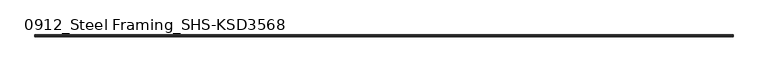
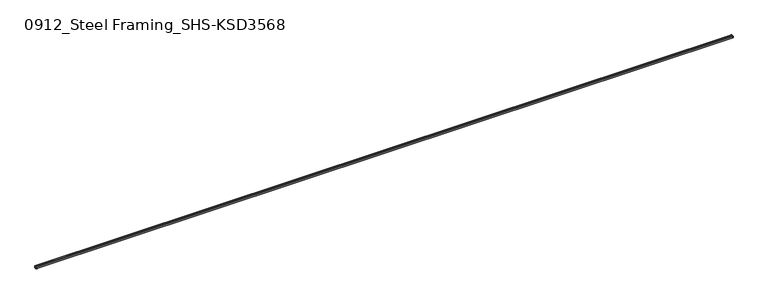
"""IFC4 building model written with IfcOpenShell, lengths in millimetres: beam geometry, 0912_Steel Framing_SHS-KSD3568 : H_SB_ASB_SHS-150x150x6."""

from ifc_helpers import new_model, si_unit, point, frame, frame_2d, origin, place, context, project, spatial, polyline, circle_curve, trimmed, segment, composite_curve, outline, extrude, source, transform, mapped, element, save


def beam_0912_steel_framing_shs_ksd3568_304e2736(model_context):
    return source(origin(), model_context, "Body", "SweptSolid", [
        extrude(outline(composite_curve([segment(polyline([(75.0, 63.0), (75.0, -63.0)]), True, "CONTINUOUS"), segment(trimmed(circle_curve(frame_2d((63.0, -63.0)), 12.0), [point((75.0, -63.0))], [point((63.0, -75.0))], False, "CARTESIAN"), True, "CONTINUOUS"), segment(polyline([(63.0, -75.0), (-63.0, -75.0)]), True, "CONTINUOUS"), segment(trimmed(circle_curve(frame_2d((-63.0, -63.0)), 12.0), [point((-63.0, -75.0))], [point((-75.0, -63.0))], False, "CARTESIAN"), True, "CONTINUOUS"), segment(polyline([(-75.0, -63.0), (-75.0, 63.0)]), True, "CONTINUOUS"), segment(trimmed(circle_curve(frame_2d((-63.0, 63.0)), 12.0), [point((-75.0, 63.0))], [point((-63.0, 75.0))], False, "CARTESIAN"), True, "CONTINUOUS"), segment(polyline([(-63.0, 75.0), (63.0, 75.0)]), True, "CONTINUOUS"), segment(trimmed(circle_curve(frame_2d((63.0, 63.0)), 12.0), [point((63.0, 75.0))], [point((75.0, 63.0))], False, "CARTESIAN"), True, "CONTINUOUS")], self_intersect=False), holes=[composite_curve([segment(trimmed(circle_curve(frame_2d((-63.0, 63.0)), 6.0), [point((-63.0, 69.0))], [point((-69.0, 63.0))], True, "CARTESIAN"), True, "CONTINUOUS"), segment(polyline([(-69.0, 63.0), (-69.0, -63.0)]), True, "CONTINUOUS"), segment(trimmed(circle_curve(frame_2d((-63.0, -63.0)), 6.0), [point((-69.0, -63.0))], [point((-63.0, -69.0))], True, "CARTESIAN"), True, "CONTINUOUS"), segment(polyline([(-63.0, -69.0), (63.0, -69.0)]), True, "CONTINUOUS"), segment(trimmed(circle_curve(frame_2d((63.0, -63.0)), 6.0), [point((63.0, -69.0))], [point((69.0, -63.0))], True, "CARTESIAN"), True, "CONTINUOUS"), segment(polyline([(69.0, -63.0), (69.0, 63.0)]), True, "CONTINUOUS"), segment(trimmed(circle_curve(frame_2d((63.0, 63.0)), 6.0), [point((69.0, 63.0))], [point((63.0, 69.0))], True, "CARTESIAN"), True, "CONTINUOUS"), segment(polyline([(63.0, 69.0), (-63.0, 69.0)]), True, "CONTINUOUS")], self_intersect=False)]), frame((-25654.5, 0.0, 0.0), z_axis=(1.0, 0.0, 0.0), x_axis=(0.0, 1.0, 0.0)), (0.0, 0.0, 1.0), 51309.0),
    ])


if __name__ == "__main__":
    model = new_model("IFC4")
    model_context = context("Model", 3, world=origin())
    ifc_project = project(units=[si_unit("LENGTHUNIT", "METRE", prefix="MILLI")], contexts=[model_context])
    site = spatial("IfcSite", under=ifc_project)
    building = spatial("IfcBuilding", under=site)
    placement = place(None, origin())
    beam_0912_steel_framing_shs_ksd3568_shape = beam_0912_steel_framing_shs_ksd3568_304e2736(model_context)
    element("IfcBeam", 1, ObjectType="0912_Steel Framing_SHS-KSD3568 : H_SB_ASB_SHS-150x150x6", at=placement, inside=building, context=model_context, shape_type="MappedRepresentation", body=[
        mapped(beam_0912_steel_framing_shs_ksd3568_shape, transform((0.0, 0.0, 0.0), x_axis=(1.0, 0.0, 0.0), y_axis=(0.0, 1.0, 0.0), z_axis=(0.0, 0.0, 1.0))),
    ])
    save(model, "model.ifc")

# Revit data of these elements
# Type "0912_Steel Framing_SHS-KSD3568 : H_SB_ASB_SHS-150x150x6"
#   H_WM Code_1 = "S01AA002-00001 | Main Steel Structure Fabrication Work | Shelter/Building | Medium Steel - Standard (90KG/M>Weight≥30KG/M) | Material: (   )"
#   H_WM Code_2 = "S03AA028-00001 | Main Steel Structure Erection Work | Shelter/Building | Medium Steel (90KG/M>Weight≥30KG/M) | Material: (   )"
#   H_WM Code_3 = "S01AA010-00001 | Main Steel Structure Fabrication Work | Shelter/Building | Steel Painting/Coating | for Non-Fireproofed Steel Surface, Surface Preparation, Primer, Second & Final Coat | Material: (   )"
#   H_Q'ty Cal Type Tag = "SB-Q2"
#   Perimeter = 0.60 m²/m
#   Nominal Weight = 26.40 kgf/m
#   Length [instance default] = 1.0000 m
#   b = 0.1500 m
#   h = 0.1500 m
#   tr = 0.0120 m
#   t = 0.0060 m
#   A = 28.36 m²
#   Structural Material [instance default] = Steel, 45-345
# Element 1 (IfcBeam, "0912_Steel Framing_SHS-KSD3568 : H_SB_ASB_SHS-150x150x6")
#   Structural Material = none
# Materials
#   "Steel, 45-345": class "Metal", colour RGB 189 187 185, transparency 0, Description = "Steel 345 MPa", Cost = 0
